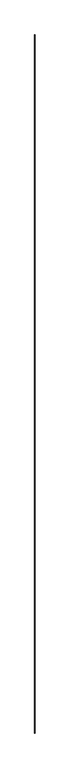
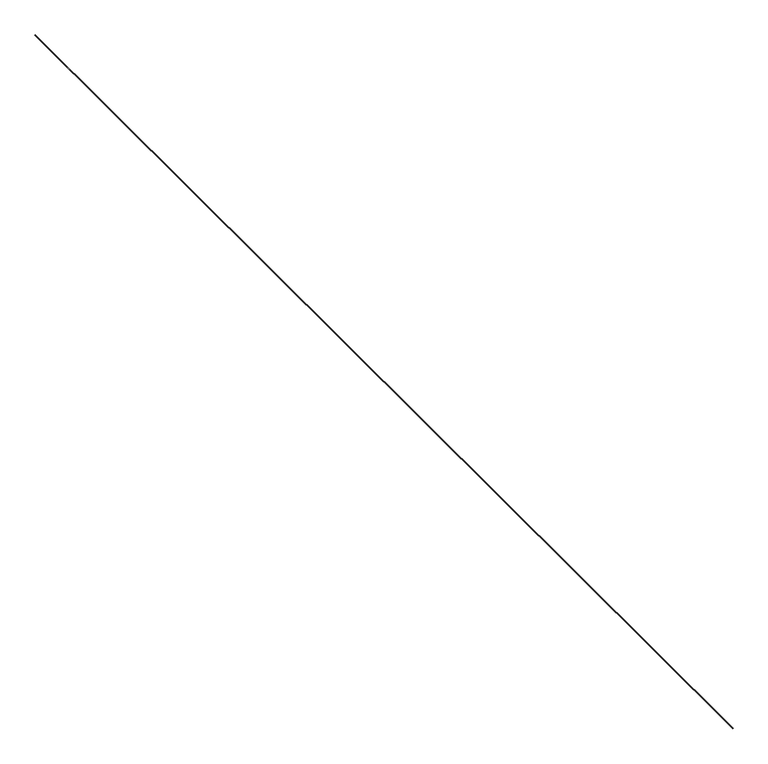
"""IFC4 building model written with IfcOpenShell, lengths in millimetres: proxy geometry, Inner panel:Inner panel:1:Inner panel:1 : Inner panel:Inner panel:300324:2:Inner panel:1:Inner panel:1 : Inner panel:Inner panel:300324:2 : Inner panel:Inner panel:1:Inner panel:1 : Inner panel:Inner panel:300324:300043:59 : Inner panel:Inner panel:1:Inner panel:1 : Inner panel:Inner panel:300324:2:Inner panel:1:Inner panel:1 : Inner panel:Inner panel:300324:2 : Inner panel:Inner panel:1:Inner panel:1 : Inner panel:Inner panel:300324:300043:308120."""

from ifc_helpers import new_model, si_unit, frame, origin, place, context, project, spatial, polyline, outline, extrude, source, transform, mapped, element, save


def generic_models_d885239a(model_context):
    return source(origin(), model_context, "Body", "SweptSolid", [
        extrude(outline(polyline([(3864.9966716, 558328.0214085), (3863.9392558, 558302.6434284), (3838.5612757, 558303.7008443), (3838.8256297, 558310.0453393), (3858.6521766, 558328.2857625), (3864.9966716, 558328.0214085)]), holes=[polyline([(3861.6922472, 558324.981338), (3859.8339876, 558325.0587654), (3841.9431277, 558308.5991744), (3841.8657002, 558306.7409148), (3860.8991853, 558305.9478529), (3861.6922472, 558324.981338)])]), frame((0.0, -579346.5018006, 0.0), z_axis=(0.0, 1.0, 0.0), x_axis=(0.0, 0.0, 1.0)), (0.0, 0.0, 1.0), 88442.8),
    ])


if __name__ == "__main__":
    model = new_model("IFC4")
    model_context = context("Model", 3, world=origin())
    ifc_project = project(units=[si_unit("LENGTHUNIT", "METRE", prefix="MILLI")], contexts=[model_context])
    site = spatial("IfcSite", under=ifc_project)
    building = spatial("IfcBuilding", under=site)
    placement = place(None, origin())
    generic_models_shape = generic_models_d885239a(model_context)
    element("IfcBuildingElementProxy", 1, Name="Inner panel:Inner panel:1:Inner panel:1 : Inner panel:Inner panel:300324:2:Inner panel:1:Inner panel:1 : Inner panel:Inner panel:300324:2 : Inner panel:Inner panel:1:Inner panel:1 : Inner panel:Inner panel:300324:300043:59 : Inner panel:Inner panel:1:Inner panel:1 : Inner panel:Inner panel:300324:2:Inner panel:1:Inner panel:1 : Inner panel:Inner panel:300324:2 : Inner panel:Inner panel:1:Inner panel:1 : Inner panel:Inner panel:300324:300043:308120", ObjectType="Inner panel:Inner panel:1:Inner panel:1 : Inner panel:Inner panel:300324:2:Inner panel:1:Inner panel:1 : Inner panel:Inner panel:300324:2 : Inner panel:Inner panel:1:Inner panel:1 : Inner panel:Inner panel:300324:300043:59 : Inner panel:Inner panel:1:Inner panel:1 : Inner panel:Inner panel:300324:2:Inner panel:1:Inner panel:1 : Inner panel:Inner panel:300324:2 : Inner panel:Inner panel:1:Inner panel:1 : Inner panel:Inner panel:300324:300043:308120", at=placement, inside=building, context=model_context, shape_type="MappedRepresentation", body=[
        mapped(generic_models_shape, transform((0.0, 0.0, 0.0), x_axis=(1.0, 0.0, 0.0), y_axis=(0.0, 1.0, 0.0), z_axis=(0.0, 0.0, 1.0))),
    ])
    save(model, "model.ifc")

# Revit data of these elements
# Type "Inner panel:Inner panel:1:Inner panel:1 : Inner panel:Inner panel:300324:2:Inner panel:1:Inner panel:1 : Inner panel:Inner panel:300324:2 : Inner panel:Inner panel:1:Inner panel:1 : Inner panel:Inner panel:300324:300043:59 : Inner panel:Inner panel:1:Inner panel:1 : Inner panel:Inner panel:300324:2:Inner panel:1:Inner panel:1 : Inner panel:Inner panel:300324:2 : Inner panel:Inner panel:1:Inner panel:1 : Inner panel:Inner panel:300324:300043:308120"
#   NameOverride = "Inner panel:Inner panel:1:Inner panel:1 : Inner panel:Inner panel:300324:2:Inner panel:1:Inner panel:1 : Inner panel:Inner panel:300324:2 : Inner panel:Inner panel:1:Inner panel:1 : Inner panel:Inner panel:300324:300043:308120"
#   ObjectTypeOverride = "Inner panel:1:Inner panel:1 : Inner panel:Inner panel:300324:2 : Inner panel:Inner panel:1:Inner panel:1 : Inner panel:Inner panel:300324:300043"
#   Reference = "Inner panel"
#   Tag = "308120"
# Element 1 (IfcBuildingElementProxy, "Inner panel:Inner panel:1:Inner panel:1 : Inner panel:Inner panel:300324:2:Inner panel:1:Inner panel:1 : Inner panel:Inner panel:300324:2 : Inner panel:Inner panel:1:Inner panel:1 : Inner panel:Inner panel:300324:300043:59 : Inner panel:Inner panel:1:Inner panel:1 : Inner panel:Inner panel:300324:2:Inner panel:1:Inner panel:1 : Inner panel:Inner panel:300324:2 : Inner panel:Inner panel:1:Inner panel:1 : Inner panel:Inner panel:300324:300043:308120")
#   Materials on its faces: "LINEAR LED LIGHTING - EXTERIOR GRADE (RUN ELEC. CONDUIT ALONG GLULAM)"
# Materials
#   "LINEAR LED LIGHTING - EXTERIOR GRADE (RUN ELEC. CONDUIT ALONG GLULAM)": class "Generic", colour RGB 120 120 120, transparency 0, Cost = 0
